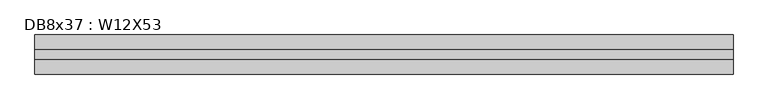
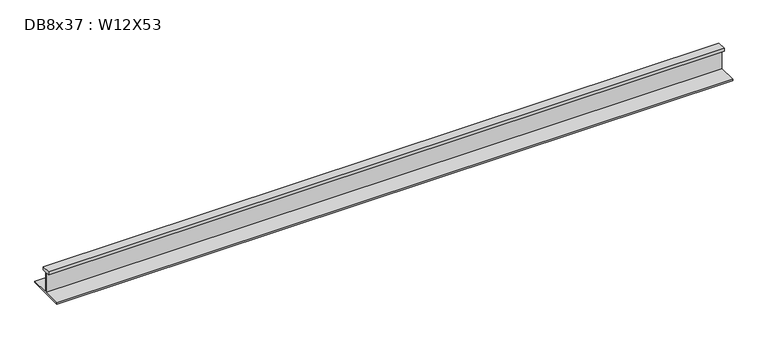
"""IFC4 building model written with IfcOpenShell, lengths in millimetres: beam geometry, DB8x37 : W12X53."""

import ifcopenshell
import ifcopenshell.guid

model = None  # the IFC model being written
_history = None  # IfcOwnerHistory: only IFC2X3 demands one
_inside = {}  # id of a spatial element -> (the spatial element, [elements in it])
_under = {}  # id of a project, library or spatial element -> (it, [spatial elements below it])
_declared = {}  # id of a project -> (the project, [libraries it declares])
_typed = {}  # id of a type object -> (the type object, [elements of that type])
_made_of = {}  # id of a material, layer set ... -> (it, [elements and type objects made of it])


def new_model(schema):
    """Start an empty IFC model of exactly this schema.

    Asked for "IFC4X3", IfcOpenShell would pick the latest addendum, in which some entities
    have other attributes; the version numbers below select the first issue.
    IFC2X3 requires an IfcOwnerHistory on every rooted entity: one is made here for all.
    """
    global model, _history
    if schema == "IFC4X3":
        model = ifcopenshell.file(schema_version=(4, 3, 0, 0))
    else:
        model = ifcopenshell.file(schema=schema)
    _inside.clear()
    _under.clear()
    _declared.clear()
    _typed.clear()
    _made_of.clear()
    _history = None
    if model.schema == "IFC2X3":
        org = make("IfcOrganization", Name="unknown")
        user = make(
            "IfcPersonAndOrganization",
            ThePerson=make("IfcPerson", FamilyName="unknown"),
            TheOrganization=org,
        )
        app = make(
            "IfcApplication",
            ApplicationDeveloper=org,
            Version="unknown",
            ApplicationFullName="unknown",
            ApplicationIdentifier="unknown",
        )
        _history = make(
            "IfcOwnerHistory",
            OwningUser=user,
            OwningApplication=app,
            ChangeAction="ADDED",
            CreationDate=0,
        )
    return model


def make(cls, **values):
    """One entity of the class cls with the attributes given. An attribute that is None is left unset."""
    return model.create_entity(
        cls, **{name: value for name, value in values.items() if value is not None}
    )


def rooted(cls, **values):
    """An entity with a GlobalId (a new one), such as an element, a storey or a relation."""
    return make(cls, GlobalId=ifcopenshell.guid.new(), OwnerHistory=_history, **values)


def si_unit(unit_type, name, prefix=None):
    """IfcSIUnit, for example si_unit("LENGTHUNIT", "METRE", prefix="MILLI")."""
    return make("IfcSIUnit", UnitType=unit_type, Prefix=prefix, Name=name)


def assignment(units):
    """IfcUnitAssignment: the units of a project."""
    return None if units is None else make("IfcUnitAssignment", Units=units)


def point(xyz):
    """IfcCartesianPoint."""
    return None if xyz is None else make("IfcCartesianPoint", Coordinates=xyz)


def direction(xyz):
    """IfcDirection."""
    return None if xyz is None else make("IfcDirection", DirectionRatios=xyz)


def frame(location, z_axis=None, x_axis=None):
    """IfcAxis2Placement3D, a coordinate frame: its origin and axes. An axis left out is left unset."""
    return make(
        "IfcAxis2Placement3D",
        Location=point(location),
        Axis=direction(z_axis),
        RefDirection=direction(x_axis),
    )


def origin():
    """The frame at (0, 0, 0) with its axes left unset."""
    return frame((0.0, 0.0, 0.0))


def place(relative_to, where):
    """IfcLocalPlacement: puts the frame where relative to a parent placement (None: the world)."""
    return make(
        "IfcLocalPlacement", PlacementRelTo=relative_to, RelativePlacement=where
    )


def context(
    kind, dimensions, precision=None, world=None, true_north=None, identifier=None
):
    """IfcGeometricRepresentationContext, for example the 3D "Model" context."""
    return make(
        "IfcGeometricRepresentationContext",
        ContextIdentifier=identifier,
        ContextType=kind,
        CoordinateSpaceDimension=dimensions,
        Precision=precision,
        WorldCoordinateSystem=world,
        TrueNorth=true_north,
    )


def project(units=None, contexts=None):
    """IfcProject with its units and contexts."""
    return rooted(
        "IfcProject",
        Name="project",
        RepresentationContexts=contexts,
        UnitsInContext=assignment(units),
    )


def spatial(cls, under=None, at=None, **own):
    """A site, building, storey or space (cls), placed at a placement, below another one or the project."""
    s = rooted(cls, ObjectPlacement=at, **own)
    if under is not None:
        _under.setdefault(under.id(), (under, []))[1].append(s)
    return s


def polyline(points):
    """IfcPolyline through the points."""
    return make("IfcPolyline", Points=[point(p) for p in points])


def outline(outer, holes=None, kind="AREA"):
    """IfcArbitraryClosedProfileDef: a profile drawn as a closed curve; with holes, ...WithVoids."""
    if holes is None:
        return make("IfcArbitraryClosedProfileDef", ProfileType=kind, OuterCurve=outer)
    return make(
        "IfcArbitraryProfileDefWithVoids",
        ProfileType=kind,
        OuterCurve=outer,
        InnerCurves=holes,
    )


def extrude(swept, where, along, depth):
    """IfcExtrudedAreaSolid: the profile swept, set in the frame where, extruded along a direction by depth."""
    return make(
        "IfcExtrudedAreaSolid",
        SweptArea=swept,
        Position=where,
        ExtrudedDirection=direction(along),
        Depth=depth,
    )


def shape(context_of_items, identifier, shape_type, items):
    """IfcShapeRepresentation: the items that make up one representation, for example the "Body"."""
    return make(
        "IfcShapeRepresentation",
        ContextOfItems=context_of_items,
        RepresentationIdentifier=identifier,
        RepresentationType=shape_type,
        Items=items,
    )


def source(mapping_origin, context_of_items, identifier, shape_type, items):
    """IfcRepresentationMap: a shape defined once, which mapped items show again and again."""
    return make(
        "IfcRepresentationMap",
        MappingOrigin=mapping_origin,
        MappedRepresentation=shape(context_of_items, identifier, shape_type, items),
    )


def transform(
    local_origin,
    x_axis=None,
    y_axis=None,
    z_axis=None,
    scale=None,
    scale2=None,
    scale3=None,
    uniform=True,
):
    """IfcCartesianTransformationOperator3D, or its non-uniform kind. x_axis, y_axis, z_axis: its Axis1, 2, 3."""
    if uniform:
        return make(
            "IfcCartesianTransformationOperator3D",
            Axis1=direction(x_axis),
            Axis2=direction(y_axis),
            LocalOrigin=point(local_origin),
            Scale=scale,
            Axis3=direction(z_axis),
        )
    return make(
        "IfcCartesianTransformationOperator3DnonUniform",
        Axis1=direction(x_axis),
        Axis2=direction(y_axis),
        LocalOrigin=point(local_origin),
        Scale=scale,
        Axis3=direction(z_axis),
        Scale2=scale2,
        Scale3=scale3,
    )


def mapped(mapping_source, mapping_target):
    """IfcMappedItem: shows the shape of a source again, moved by a transform."""
    return make(
        "IfcMappedItem", MappingSource=mapping_source, MappingTarget=mapping_target
    )


def made_of(thing, what):
    """Note that an element or type object is made of a material, layer set ...; save() writes the relation."""
    if what is not None:
        _made_of.setdefault(what.id(), (what, []))[1].append(thing)
    return thing


def element(
    cls,
    number,
    at=None,
    inside=None,
    cuts=None,
    type_object=None,
    material=None,
    context=None,
    identifier="Body",
    shape_type=None,
    held_by="IfcProductDefinitionShape",
    body=None,
    shapes=None,
    **own,
):
    """One element of the class cls, such as IfcWall. Its Tag is "e" and its number.

    at: its placement. inside: the storey or other place that contains it. cuts: it is an
    opening in that element (IfcRelVoidsElement). A single representation is given by context,
    identifier, shape_type and body (its items); several are given by shapes. held_by: the class
    of the entity that holds the representations. save() writes the other relations.
    """
    e = rooted(cls, Tag="e%d" % number, ObjectPlacement=at, **own)
    if body is not None:
        shapes = [shape(context, identifier, shape_type, body)]
    if shapes is not None:
        e.Representation = make(held_by, Representations=shapes)
    if inside is not None:
        _inside.setdefault(inside.id(), (inside, []))[1].append(e)
    if cuts is not None:
        rooted(
            "IfcRelVoidsElement", RelatingBuildingElement=cuts, RelatedOpeningElement=e
        )
    if type_object is not None:
        _typed.setdefault(type_object.id(), (type_object, []))[1].append(e)
    return made_of(e, material)


def aggregate(whole, parts):
    """IfcRelAggregates: a whole, such as a stair, and the parts it consists of."""
    return rooted("IfcRelAggregates", RelatingObject=whole, RelatedObjects=parts)


def save(model, path):
    """Write the relations noted so far, then the file.

    IfcRelAggregates (storeys below a building ...), IfcRelContainedInSpatialStructure (elements
    in a storey), IfcRelDefinesByType, IfcRelAssociatesMaterial and IfcRelDeclares: one each for
    every whole, place, type object, material and project.
    """
    for whole, parts in _under.values():
        aggregate(whole, parts)
    for where, things in _inside.values():
        rooted(
            "IfcRelContainedInSpatialStructure",
            RelatedElements=things,
            RelatingStructure=where,
        )
    for kind, things in _typed.values():
        rooted("IfcRelDefinesByType", RelatedObjects=things, RelatingType=kind)
    for what, things in _made_of.values():
        rooted("IfcRelAssociatesMaterial", RelatedObjects=things, RelatingMaterial=what)
    for by, libraries in _declared.values():
        rooted("IfcRelDeclares", RelatingContext=by, RelatedDefinitions=libraries)
    model.write(path)


def db8x37_w12x53_7e8dff65(model_context):
    return source(origin(), model_context, "Body", "SweptSolid", [
        extrude(outline(polyline([(38.1, 145.415), (38.1, 120.015), (2.921, 120.015), (2.921, -48.4505), (152.4, -48.4505), (152.4, -58.1025), (-152.4, -58.1025), (-152.4, -48.4505), (-2.921, -48.4505), (-2.921, 120.015), (-38.1, 120.015), (-38.1, 145.415), (38.1, 145.415)])), frame((-2793.873, 0.0, 0.0), z_axis=(1.0, 0.0, 0.0), x_axis=(0.0, 1.0, 0.0)), (0.0, 0.0, 1.0), 5438.902),
    ])


if __name__ == "__main__":
    model = new_model("IFC4")
    model_context = context("Model", 3, world=origin())
    ifc_project = project(units=[si_unit("LENGTHUNIT", "METRE", prefix="MILLI")], contexts=[model_context])
    site = spatial("IfcSite", under=ifc_project)
    building = spatial("IfcBuilding", under=site)
    placement = place(None, origin())
    db8x37_w12x53_shape = db8x37_w12x53_7e8dff65(model_context)
    element("IfcBeam", 1, ObjectType="DB8x37 : W12X53", at=placement, inside=building, context=model_context, shape_type="MappedRepresentation", body=[
        mapped(db8x37_w12x53_shape, transform((0.0, 0.0, 0.0), x_axis=(1.0, 0.0, 0.0), y_axis=(0.0, 1.0, 0.0), z_axis=(0.0, 0.0, 1.0))),
    ])
    save(model, "model.ifc")

# Revit data of these elements
# Type "DB8x37 : W12X53"
#   Assembly Code = "B10"
#   W = 53
#   Length [instance default] = 5' - 0"
#   bf = 0' - 10"
#   d = 1' - 0.1"
#   k = 0' - 1 3/8"
#   k2 = 0' - 0.8"
#   tf = 0' - 0.575"
#   tw = 0' - 0.345"
#   A = 0.108333 SF
#   Structural Material [instance default] = Steel ASTM A992
# Element 1 (IfcBeam, "DB8x37 : W12X53")
#   Materials on its faces: "Steel ASTM A992"
# Materials
#   "Steel ASTM A992": class "Metal", colour RGB 199 199 199, transparency 0, Description = "Structural steel 50ksi", Cost = 0
